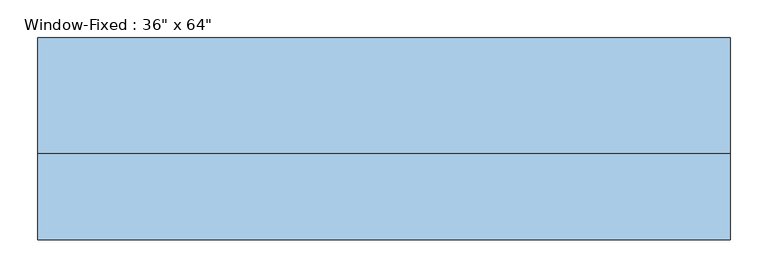
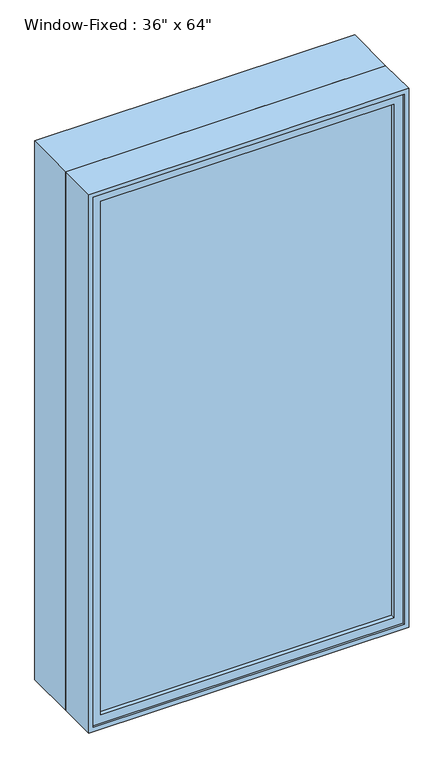
"""IFC4 building model written with IfcOpenShell, lengths in millimetres: window geometry."""

from ifc_helpers import new_model, si_unit, frame, origin, place, context, project, spatial, polyline, outline, extrude, faceted_brep, source, transform, mapped, element, save


def window_b05dfed1(model_context):
    return source(origin(), model_context, "Body", "SolidModel", [
        extrude(outline(polyline([(419.1, -79.375), (-419.1, -79.375), (-419.1, -73.025), (419.1, -73.025), (419.1, -79.375)])), frame((0.0, 0.0, 952.5), z_axis=(0.0, 0.0, 1.0), x_axis=(1.0, 0.0, 0.0)), (0.0, 0.0, 1.0), 1549.4),
        extrude(outline(polyline([(-419.1, -60.325), (419.1, -60.325), (419.1, -66.675), (-419.1, -66.675), (-419.1, -60.325)])), frame((0.0, 0.0, 952.5), z_axis=(0.0, 0.0, 1.0), x_axis=(1.0, 0.0, 0.0)), (0.0, 0.0, 1.0), 1549.4),
        extrude(outline(polyline([(927.1, -444.5), (927.1, 444.5), (2527.3, 444.5), (2527.3, -444.5), (927.1, -444.5)]), holes=[polyline([(952.5, 419.1), (952.5, -419.1), (2501.9, -419.1), (2501.9, 419.1), (952.5, 419.1)])]), frame((0.0, -92.075, 0.0), z_axis=(0.0, 1.0, 0.0), x_axis=(0.0, 0.0, 1.0)), (0.0, 0.0, 1.0), 44.45),
        extrude(outline(polyline([(2540.0, -457.2), (914.4, -457.2), (914.4, 457.2), (2540.0, 457.2), (2540.0, -457.2)]), holes=[polyline([(2527.3, 444.5), (927.1, 444.5), (927.1, -444.5), (2527.3, -444.5), (2527.3, 444.5)])]), frame((0.0, 15.875, 0.0), z_axis=(0.0, 1.0, 0.0), x_axis=(0.0, 0.0, 1.0)), (0.0, 0.0, 1.0), 152.4),
        faceted_brep([(457.2, 15.875, 2540.0), (-457.2, 15.875, 2540.0), (-457.2, -98.425, 2540.0), (457.2, -98.425, 2540.0), (-457.2, 15.875, 914.4), (-457.2, -98.425, 914.4), (457.2, 15.875, 914.4), (457.2, -98.425, 914.4), (425.45, 15.875, 2508.25), (-425.45, 15.875, 2508.25), (-425.45, 15.875, 946.15), (425.45, 15.875, 946.15), (-444.5, -98.425, 2527.3), (444.5, -98.425, 2527.3), (444.5, -98.425, 927.1), (-444.5, -98.425, 927.1), (425.45, -47.625, 2508.25), (-425.45, -47.625, 2508.25), (-444.5, -47.625, 2527.3), (444.5, -47.625, 2527.3), (-425.45, -47.625, 946.15), (-444.5, -47.625, 927.1), (425.45, -47.625, 946.15), (444.5, -47.625, 927.1)], [[[0, 1, 2, 3]], [[1, 4, 5, 2]], [[4, 6, 7, 5]], [[1, 0, 6, 4], [8, 9, 10, 11]], [[6, 0, 3, 7]], [[3, 2, 5, 7], [12, 13, 14, 15]], [[16, 17, 9, 8]], [[13, 12, 18, 19]], [[17, 20, 10, 9]], [[12, 15, 21, 18]], [[20, 22, 11, 10]], [[15, 14, 23, 21]], [[22, 16, 8, 11]], [[19, 18, 21, 23], [17, 16, 22, 20]], [[14, 13, 19, 23]]]),
    ])


if __name__ == "__main__":
    model = new_model("IFC4")
    model_context = context("Model", 3, world=origin())
    ifc_project = project(units=[si_unit("LENGTHUNIT", "METRE", prefix="MILLI")], contexts=[model_context])
    site = spatial("IfcSite", under=ifc_project)
    building = spatial("IfcBuilding", under=site)
    placement = place(None, origin())
    window_shape = window_b05dfed1(model_context)
    element("IfcWindow", 1, ObjectType="Window-Fixed : 36\" x 64\"", at=placement, inside=building, context=model_context, shape_type="MappedRepresentation", body=[
        mapped(window_shape, transform((0.0, 0.0, 0.0), x_axis=(1.0, 0.0, 0.0), y_axis=(0.0, 1.0, 0.0), z_axis=(0.0, 0.0, 1.0))),
    ])
    save(model, "model.ifc")

# Revit data of these elements
# Type "Window-Fixed : 36\" x 64\""
#   Type Mark = "23"
#   Fire Rating = "0.5h"
#   Assembly Code = "B2020100"
#   Analytic Construction = "Double glazing - domestic"
#   Window Inset [instance default] = 0' - 0"
#   Wall Thickness [instance default] = 0' - 6"
#   Visual Light Transmittance = 0.81
#   Thermal Resistance (R) = 1.8146 (h·ft²·°F)/BTU
#   Solar Heat Gain Coefficient = 0.76
#   Rough Width = 3' - 0 1/2"
#   Rough Height = 5' - 4 1/2"
#   Interior Wall Closure [instance default] = 0' - 2 1/4"
#   Height = 5' - 4"
#   Heat Transfer Coefficient (U) = 0.5511 BTU/(h·ft²·°F)
#   Frame Extension [instance default] = 0' - 0 1/4"
#   Exterior Wall Closure [instance default] = 0' - 1 1/4"
#   Extension Jamb [instance default] = 0' - 2 1/4"
#   Default Sill Height = 3' - 0"
#   Width = 3' - 0"
#   Muntin Visibility = yes
#   Interior Trim Visibility [instance default] = yes
#   Exterior Trim Visibility [instance default] = yes
#   Extension Jamb Visibility [instance default] = yes
#   Muntin Pattern = Muntin Pattern_2x2 : Muntin Pattern_2x2
#   Interior Trim Material = Wood - Stained
#   Interior Trim = Trim-Window-Interior-Flat : Picture Frame
#   Interior Frame Material = Wood - Stained
#   Glass Panel Material = Glass
#   Exterior Trim Material = Clad - White
#   Exterior Trim = Trim-Window-Exterior-Flat : with Sill
#   Exterior Frame Material = Clad - White
#   Wall Closure = (empty or 0)
# Element 1 (IfcWindow, "Window-Fixed : 36\" x 64\"")
#   Window Inset = 0' - 3 1/2"
#   Wall Thickness = 1' - 1 1/4"
#   Exterior Wall Closure = 0' - 5 1/2"
#   Extension Jamb = 0' - 6"
#   Exterior Trim Visibility = no
#   Materials on its faces: "Wood - Stained", "Glass", "Clad - White"
# Materials
#   "Wood - Stained": class "Wood", colour RGB 224 178 126, transparency 0, Cost = 0
#   "Glass": class "Glass", colour RGB 0 128 192, transparency 0.75, Description = "Soda Lime Glass", Cost = 0
#   "Clad - White": class "Wood", colour RGB 242 242 238, transparency 0, Cost = 0
